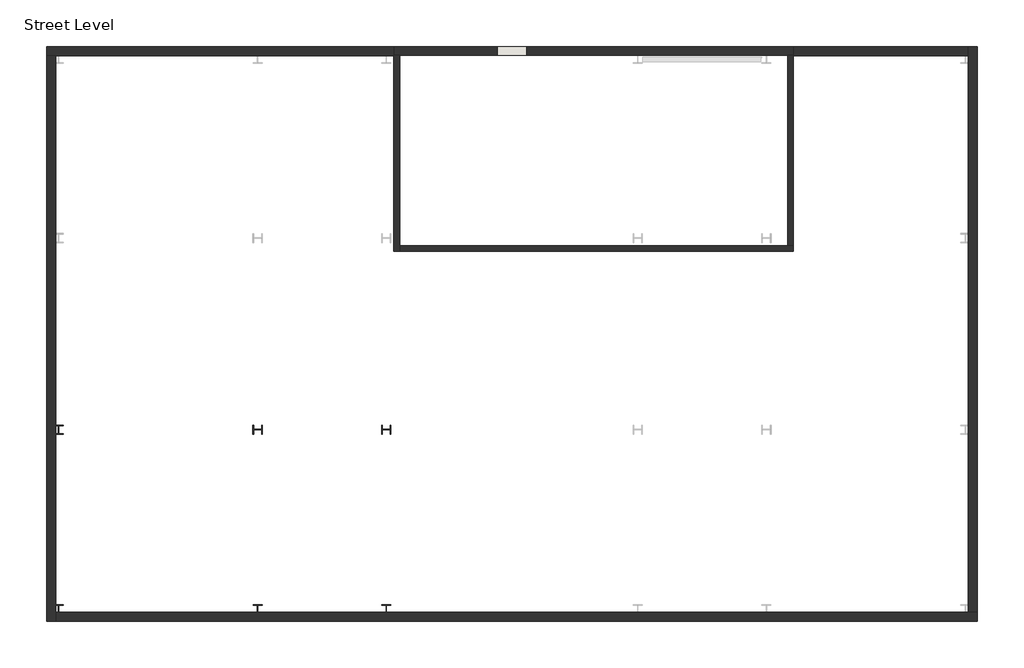
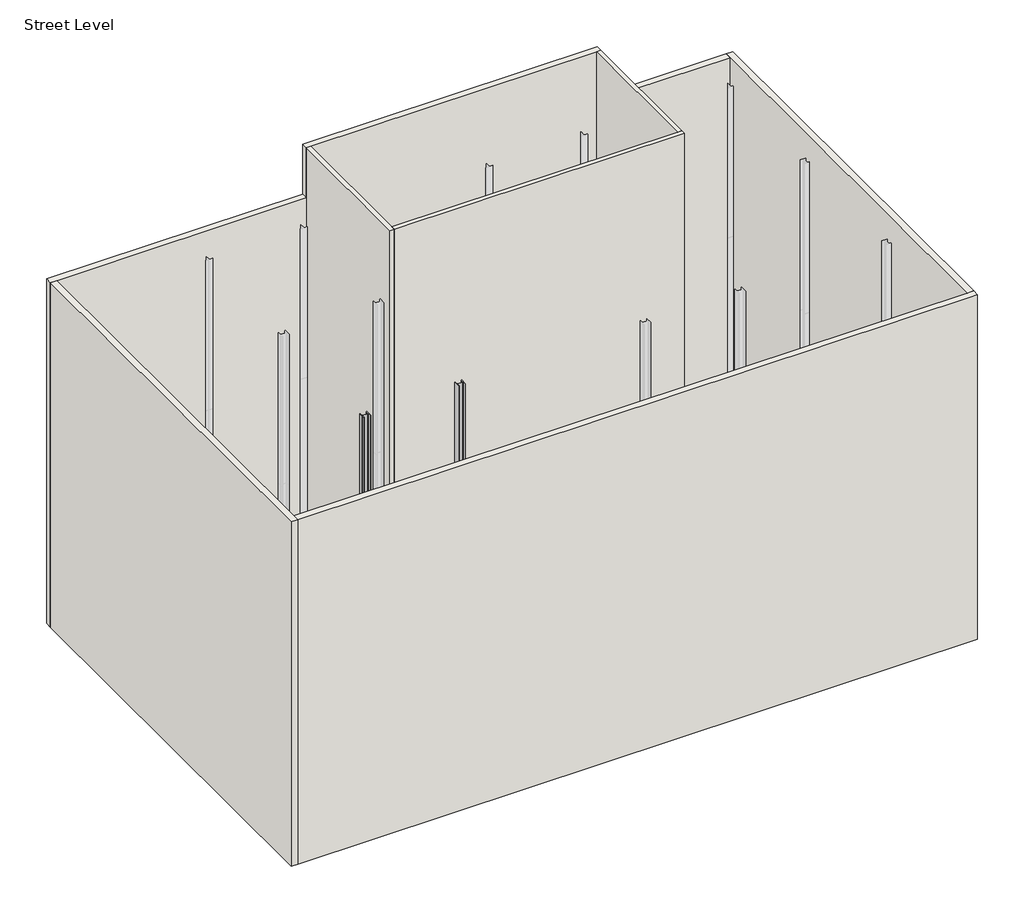
# One storey, part 1 of 3: 9 walls, 6 columns.
"""IFC4 building model written with IfcOpenShell, lengths in millimetres."""

from ifc_helpers import new_model, si_unit, point, frame, frame_2d, origin, place, context, project, spatial, polyline, circle_curve, trimmed, segment, composite_curve, outline, extrude, faceted_brep, element, save

model = new_model("IFC4")

# Units and contexts
model_context = context("Model", 3, world=origin())
ifc_project = project(units=[si_unit("LENGTHUNIT", "METRE", prefix="MILLI")], contexts=[model_context])

# Site, building, storey
site = spatial("IfcSite", under=ifc_project)
building = spatial("IfcBuilding", under=site)
storey = spatial("IfcBuildingStorey", under=building, Name="Street Level", Elevation=-914.4)

# Columns
placement = place(None, origin())
element("IfcColumn", 1, ObjectType="W-Wide Flange-Column : W12X87", at=placement, inside=storey, context=model_context, shape_type="SweptSolid", body=[
    extrude(outline(composite_curve([segment(polyline([(-9643.0622732, -3562.1684696), (-9663.6362732, -3562.1684696), (-9663.6362732, -3437.3274696)]), True, "CONTINUOUS"), segment(trimmed(circle_curve(frame_2d((-9685.9247732, -3437.3274696)), 22.2885), [point((-9663.6362732, -3437.3274696))], [point((-9685.9247732, -3415.0389696))], True, "CARTESIAN"), True, "CONTINUOUS"), segment(polyline([(-9685.9247732, -3415.0389696), (-9917.6997732, -3415.0389696)]), True, "CONTINUOUS"), segment(trimmed(circle_curve(frame_2d((-9917.6997732, -3437.3274696)), 22.2885), [point((-9917.6997732, -3415.0389696))], [point((-9939.9882732, -3437.3274696))], True, "CARTESIAN"), True, "CONTINUOUS"), segment(polyline([(-9939.9882732, -3437.3274696), (-9939.9882732, -3562.1684696), (-9960.5622732, -3562.1684696), (-9960.5622732, -3254.8284696), (-9939.9882732, -3254.8284696), (-9939.9882732, -3379.6694696)]), True, "CONTINUOUS"), segment(trimmed(circle_curve(frame_2d((-9917.6997732, -3379.6694696)), 22.2885), [point((-9939.9882732, -3379.6694696))], [point((-9917.6997732, -3401.9579696))], True, "CARTESIAN"), True, "CONTINUOUS"), segment(polyline([(-9917.6997732, -3401.9579696), (-9685.9247732, -3401.9579696)]), True, "CONTINUOUS"), segment(trimmed(circle_curve(frame_2d((-9685.9247732, -3379.6694696)), 22.2885), [point((-9685.9247732, -3401.9579696))], [point((-9663.6362732, -3379.6694696))], True, "CARTESIAN"), True, "CONTINUOUS"), segment(polyline([(-9663.6362732, -3379.6694696), (-9663.6362732, -3254.8284696), (-9643.0622732, -3254.8284696), (-9643.0622732, -3562.1684696)]), True, "CONTINUOUS")], self_intersect=False)), frame((0.0, 0.0, 7315.2), z_axis=(0.0, 0.0, 1.0), x_axis=(1.0, 0.0, 0.0)), (0.0, 0.0, 1.0), 7315.2),
    extrude(outline(composite_curve([segment(polyline([(-9643.0622732, -3562.1684696), (-9663.6362732, -3562.1684696), (-9663.6362732, -3437.3274696)]), True, "CONTINUOUS"), segment(trimmed(circle_curve(frame_2d((-9685.9247732, -3437.3274696)), 22.2885), [point((-9663.6362732, -3437.3274696))], [point((-9685.9247732, -3415.0389696))], True, "CARTESIAN"), True, "CONTINUOUS"), segment(polyline([(-9685.9247732, -3415.0389696), (-9917.6997732, -3415.0389696)]), True, "CONTINUOUS"), segment(trimmed(circle_curve(frame_2d((-9917.6997732, -3437.3274696)), 22.2885), [point((-9917.6997732, -3415.0389696))], [point((-9939.9882732, -3437.3274696))], True, "CARTESIAN"), True, "CONTINUOUS"), segment(polyline([(-9939.9882732, -3437.3274696), (-9939.9882732, -3562.1684696), (-9960.5622732, -3562.1684696), (-9960.5622732, -3254.8284696), (-9939.9882732, -3254.8284696), (-9939.9882732, -3379.6694696)]), True, "CONTINUOUS"), segment(trimmed(circle_curve(frame_2d((-9917.6997732, -3379.6694696)), 22.2885), [point((-9939.9882732, -3379.6694696))], [point((-9917.6997732, -3401.9579696))], True, "CARTESIAN"), True, "CONTINUOUS"), segment(polyline([(-9917.6997732, -3401.9579696), (-9685.9247732, -3401.9579696)]), True, "CONTINUOUS"), segment(trimmed(circle_curve(frame_2d((-9685.9247732, -3379.6694696)), 22.2885), [point((-9685.9247732, -3401.9579696))], [point((-9663.6362732, -3379.6694696))], True, "CARTESIAN"), True, "CONTINUOUS"), segment(polyline([(-9663.6362732, -3379.6694696), (-9663.6362732, -3254.8284696), (-9643.0622732, -3254.8284696), (-9643.0622732, -3562.1684696)]), True, "CONTINUOUS")], self_intersect=False)), frame((0.0, 0.0, -914.4), z_axis=(0.0, 0.0, 1.0), x_axis=(1.0, 0.0, 0.0)), (0.0, 0.0, 1.0), 8229.6),
])
element("IfcColumn", 2, ObjectType="W-Wide Flange-Column : W12X87", at=placement, inside=storey, context=model_context, shape_type="SweptSolid", body=[
    extrude(outline(composite_curve([segment(polyline([(-5274.2622732, -3562.1684696), (-5294.8362732, -3562.1684696), (-5294.8362732, -3437.3274696)]), True, "CONTINUOUS"), segment(trimmed(circle_curve(frame_2d((-5317.1247732, -3437.3274696)), 22.2885), [point((-5294.8362732, -3437.3274696))], [point((-5317.1247732, -3415.0389696))], True, "CARTESIAN"), True, "CONTINUOUS"), segment(polyline([(-5317.1247732, -3415.0389696), (-5548.8997732, -3415.0389696)]), True, "CONTINUOUS"), segment(trimmed(circle_curve(frame_2d((-5548.8997732, -3437.3274696)), 22.2885), [point((-5548.8997732, -3415.0389696))], [point((-5571.1882732, -3437.3274696))], True, "CARTESIAN"), True, "CONTINUOUS"), segment(polyline([(-5571.1882732, -3437.3274696), (-5571.1882732, -3562.1684696), (-5591.7622732, -3562.1684696), (-5591.7622732, -3254.8284696), (-5571.1882732, -3254.8284696), (-5571.1882732, -3379.6694696)]), True, "CONTINUOUS"), segment(trimmed(circle_curve(frame_2d((-5548.8997732, -3379.6694696)), 22.2885), [point((-5571.1882732, -3379.6694696))], [point((-5548.8997732, -3401.9579696))], True, "CARTESIAN"), True, "CONTINUOUS"), segment(polyline([(-5548.8997732, -3401.9579696), (-5317.1247732, -3401.9579696)]), True, "CONTINUOUS"), segment(trimmed(circle_curve(frame_2d((-5317.1247732, -3379.6694696)), 22.2885), [point((-5317.1247732, -3401.9579696))], [point((-5294.8362732, -3379.6694696))], True, "CARTESIAN"), True, "CONTINUOUS"), segment(polyline([(-5294.8362732, -3379.6694696), (-5294.8362732, -3254.8284696), (-5274.2622732, -3254.8284696), (-5274.2622732, -3562.1684696)]), True, "CONTINUOUS")], self_intersect=False)), frame((0.0, 0.0, 7315.2), z_axis=(0.0, 0.0, 1.0), x_axis=(1.0, 0.0, 0.0)), (0.0, 0.0, 1.0), 7315.2),
    extrude(outline(composite_curve([segment(polyline([(-5274.2622732, -3562.1684696), (-5294.8362732, -3562.1684696), (-5294.8362732, -3437.3274696)]), True, "CONTINUOUS"), segment(trimmed(circle_curve(frame_2d((-5317.1247732, -3437.3274696)), 22.2885), [point((-5294.8362732, -3437.3274696))], [point((-5317.1247732, -3415.0389696))], True, "CARTESIAN"), True, "CONTINUOUS"), segment(polyline([(-5317.1247732, -3415.0389696), (-5548.8997732, -3415.0389696)]), True, "CONTINUOUS"), segment(trimmed(circle_curve(frame_2d((-5548.8997732, -3437.3274696)), 22.2885), [point((-5548.8997732, -3415.0389696))], [point((-5571.1882732, -3437.3274696))], True, "CARTESIAN"), True, "CONTINUOUS"), segment(polyline([(-5571.1882732, -3437.3274696), (-5571.1882732, -3562.1684696), (-5591.7622732, -3562.1684696), (-5591.7622732, -3254.8284696), (-5571.1882732, -3254.8284696), (-5571.1882732, -3379.6694696)]), True, "CONTINUOUS"), segment(trimmed(circle_curve(frame_2d((-5548.8997732, -3379.6694696)), 22.2885), [point((-5571.1882732, -3379.6694696))], [point((-5548.8997732, -3401.9579696))], True, "CARTESIAN"), True, "CONTINUOUS"), segment(polyline([(-5548.8997732, -3401.9579696), (-5317.1247732, -3401.9579696)]), True, "CONTINUOUS"), segment(trimmed(circle_curve(frame_2d((-5317.1247732, -3379.6694696)), 22.2885), [point((-5317.1247732, -3401.9579696))], [point((-5294.8362732, -3379.6694696))], True, "CARTESIAN"), True, "CONTINUOUS"), segment(polyline([(-5294.8362732, -3379.6694696), (-5294.8362732, -3254.8284696), (-5274.2622732, -3254.8284696), (-5274.2622732, -3562.1684696)]), True, "CONTINUOUS")], self_intersect=False)), frame((0.0, 0.0, -914.4), z_axis=(0.0, 0.0, 1.0), x_axis=(1.0, 0.0, 0.0)), (0.0, 0.0, 1.0), 8229.6),
])
element("IfcColumn", 3, ObjectType="W-Wide Flange-Column : W12X87", at=placement, inside=storey, context=model_context, shape_type="SweptSolid", body=[
    extrude(outline(composite_curve([segment(polyline([(-5279.3422732, -9345.7484696), (-5279.3422732, -9366.3224696), (-5404.1832732, -9366.3224696)]), True, "CONTINUOUS"), segment(trimmed(circle_curve(frame_2d((-5404.1832732, -9388.6109696)), 22.2885), [point((-5404.1832732, -9366.3224696))], [point((-5426.4717732, -9388.6109696))], True, "CARTESIAN"), True, "CONTINUOUS"), segment(polyline([(-5426.4717732, -9388.6109696), (-5426.4717732, -9620.3859696)]), True, "CONTINUOUS"), segment(trimmed(circle_curve(frame_2d((-5404.1832732, -9620.3859696)), 22.2885), [point((-5426.4717732, -9620.3859696))], [point((-5404.1832732, -9642.6744696))], True, "CARTESIAN"), True, "CONTINUOUS"), segment(polyline([(-5404.1832732, -9642.6744696), (-5279.3422732, -9642.6744696), (-5279.3422732, -9663.2484696), (-5586.6822732, -9663.2484696), (-5586.6822732, -9642.6744696), (-5461.8412732, -9642.6744696)]), True, "CONTINUOUS"), segment(trimmed(circle_curve(frame_2d((-5461.8412732, -9620.3859696)), 22.2885), [point((-5461.8412732, -9642.6744696))], [point((-5439.5527732, -9620.3859696))], True, "CARTESIAN"), True, "CONTINUOUS"), segment(polyline([(-5439.5527732, -9620.3859696), (-5439.5527732, -9388.6109696)]), True, "CONTINUOUS"), segment(trimmed(circle_curve(frame_2d((-5461.8412732, -9388.6109696)), 22.2885), [point((-5439.5527732, -9388.6109696))], [point((-5461.8412732, -9366.3224696))], True, "CARTESIAN"), True, "CONTINUOUS"), segment(polyline([(-5461.8412732, -9366.3224696), (-5586.6822732, -9366.3224696), (-5586.6822732, -9345.7484696), (-5279.3422732, -9345.7484696)]), True, "CONTINUOUS")], self_intersect=False)), frame((0.0, 0.0, 7315.2), z_axis=(0.0, 0.0, 1.0), x_axis=(1.0, 0.0, 0.0)), (0.0, 0.0, 1.0), 7315.2),
    extrude(outline(composite_curve([segment(polyline([(-5279.3422732, -9345.7484696), (-5279.3422732, -9366.3224696), (-5404.1832732, -9366.3224696)]), True, "CONTINUOUS"), segment(trimmed(circle_curve(frame_2d((-5404.1832732, -9388.6109696)), 22.2885), [point((-5404.1832732, -9366.3224696))], [point((-5426.4717732, -9388.6109696))], True, "CARTESIAN"), True, "CONTINUOUS"), segment(polyline([(-5426.4717732, -9388.6109696), (-5426.4717732, -9620.3859696)]), True, "CONTINUOUS"), segment(trimmed(circle_curve(frame_2d((-5404.1832732, -9620.3859696)), 22.2885), [point((-5426.4717732, -9620.3859696))], [point((-5404.1832732, -9642.6744696))], True, "CARTESIAN"), True, "CONTINUOUS"), segment(polyline([(-5404.1832732, -9642.6744696), (-5279.3422732, -9642.6744696), (-5279.3422732, -9663.2484696), (-5586.6822732, -9663.2484696), (-5586.6822732, -9642.6744696), (-5461.8412732, -9642.6744696)]), True, "CONTINUOUS"), segment(trimmed(circle_curve(frame_2d((-5461.8412732, -9620.3859696)), 22.2885), [point((-5461.8412732, -9642.6744696))], [point((-5439.5527732, -9620.3859696))], True, "CARTESIAN"), True, "CONTINUOUS"), segment(polyline([(-5439.5527732, -9620.3859696), (-5439.5527732, -9388.6109696)]), True, "CONTINUOUS"), segment(trimmed(circle_curve(frame_2d((-5461.8412732, -9388.6109696)), 22.2885), [point((-5439.5527732, -9388.6109696))], [point((-5461.8412732, -9366.3224696))], True, "CARTESIAN"), True, "CONTINUOUS"), segment(polyline([(-5461.8412732, -9366.3224696), (-5586.6822732, -9366.3224696), (-5586.6822732, -9345.7484696), (-5279.3422732, -9345.7484696)]), True, "CONTINUOUS")], self_intersect=False)), frame((0.0, 0.0, -914.4), z_axis=(0.0, 0.0, 1.0), x_axis=(1.0, 0.0, 0.0)), (0.0, 0.0, 1.0), 8229.6),
])
element("IfcColumn", 4, ObjectType="W-Wide Flange-Column : W12X87", at=placement, inside=storey, context=model_context, shape_type="SweptSolid", body=[
    extrude(outline(composite_curve([segment(polyline([(-9648.1422732, -9345.7484696), (-9648.1422732, -9366.3224696), (-9772.9832732, -9366.3224696)]), True, "CONTINUOUS"), segment(trimmed(circle_curve(frame_2d((-9772.9832732, -9388.6109696)), 22.2885), [point((-9772.9832732, -9366.3224696))], [point((-9795.2717732, -9388.6109696))], True, "CARTESIAN"), True, "CONTINUOUS"), segment(polyline([(-9795.2717732, -9388.6109696), (-9795.2717732, -9620.3859696)]), True, "CONTINUOUS"), segment(trimmed(circle_curve(frame_2d((-9772.9832732, -9620.3859696)), 22.2885), [point((-9795.2717732, -9620.3859696))], [point((-9772.9832732, -9642.6744696))], True, "CARTESIAN"), True, "CONTINUOUS"), segment(polyline([(-9772.9832732, -9642.6744696), (-9648.1422732, -9642.6744696), (-9648.1422732, -9663.2484696), (-9955.4822732, -9663.2484696), (-9955.4822732, -9642.6744696), (-9830.6412732, -9642.6744696)]), True, "CONTINUOUS"), segment(trimmed(circle_curve(frame_2d((-9830.6412732, -9620.3859696)), 22.2885), [point((-9830.6412732, -9642.6744696))], [point((-9808.3527732, -9620.3859696))], True, "CARTESIAN"), True, "CONTINUOUS"), segment(polyline([(-9808.3527732, -9620.3859696), (-9808.3527732, -9388.6109696)]), True, "CONTINUOUS"), segment(trimmed(circle_curve(frame_2d((-9830.6412732, -9388.6109696)), 22.2885), [point((-9808.3527732, -9388.6109696))], [point((-9830.6412732, -9366.3224696))], True, "CARTESIAN"), True, "CONTINUOUS"), segment(polyline([(-9830.6412732, -9366.3224696), (-9955.4822732, -9366.3224696), (-9955.4822732, -9345.7484696), (-9648.1422732, -9345.7484696)]), True, "CONTINUOUS")], self_intersect=False)), frame((0.0, 0.0, 7315.2), z_axis=(0.0, 0.0, 1.0), x_axis=(1.0, 0.0, 0.0)), (0.0, 0.0, 1.0), 7315.2),
    extrude(outline(composite_curve([segment(polyline([(-9648.1422732, -9345.7484696), (-9648.1422732, -9366.3224696), (-9772.9832732, -9366.3224696)]), True, "CONTINUOUS"), segment(trimmed(circle_curve(frame_2d((-9772.9832732, -9388.6109696)), 22.2885), [point((-9772.9832732, -9366.3224696))], [point((-9795.2717732, -9388.6109696))], True, "CARTESIAN"), True, "CONTINUOUS"), segment(polyline([(-9795.2717732, -9388.6109696), (-9795.2717732, -9620.3859696)]), True, "CONTINUOUS"), segment(trimmed(circle_curve(frame_2d((-9772.9832732, -9620.3859696)), 22.2885), [point((-9795.2717732, -9620.3859696))], [point((-9772.9832732, -9642.6744696))], True, "CARTESIAN"), True, "CONTINUOUS"), segment(polyline([(-9772.9832732, -9642.6744696), (-9648.1422732, -9642.6744696), (-9648.1422732, -9663.2484696), (-9955.4822732, -9663.2484696), (-9955.4822732, -9642.6744696), (-9830.6412732, -9642.6744696)]), True, "CONTINUOUS"), segment(trimmed(circle_curve(frame_2d((-9830.6412732, -9620.3859696)), 22.2885), [point((-9830.6412732, -9642.6744696))], [point((-9808.3527732, -9620.3859696))], True, "CARTESIAN"), True, "CONTINUOUS"), segment(polyline([(-9808.3527732, -9620.3859696), (-9808.3527732, -9388.6109696)]), True, "CONTINUOUS"), segment(trimmed(circle_curve(frame_2d((-9830.6412732, -9388.6109696)), 22.2885), [point((-9808.3527732, -9388.6109696))], [point((-9830.6412732, -9366.3224696))], True, "CARTESIAN"), True, "CONTINUOUS"), segment(polyline([(-9830.6412732, -9366.3224696), (-9955.4822732, -9366.3224696), (-9955.4822732, -9345.7484696), (-9648.1422732, -9345.7484696)]), True, "CONTINUOUS")], self_intersect=False)), frame((0.0, 0.0, -914.4), z_axis=(0.0, 0.0, 1.0), x_axis=(1.0, 0.0, 0.0)), (0.0, 0.0, 1.0), 8229.6),
])
element("IfcColumn", 5, ObjectType="W-Wide Flange-Column : W12X87", at=placement, inside=storey, context=model_context, shape_type="SweptSolid", body=[
    extrude(outline(composite_curve([segment(polyline([(-16404.5422732, -9345.7484696), (-16404.5422732, -9366.3224696), (-16529.3832732, -9366.3224696)]), True, "CONTINUOUS"), segment(trimmed(circle_curve(frame_2d((-16529.3832732, -9388.6109696)), 22.2885), [point((-16529.3832732, -9366.3224696))], [point((-16551.6717732, -9388.6109696))], True, "CARTESIAN"), True, "CONTINUOUS"), segment(polyline([(-16551.6717732, -9388.6109696), (-16551.6717732, -9620.3859696)]), True, "CONTINUOUS"), segment(trimmed(circle_curve(frame_2d((-16529.3832732, -9620.3859696)), 22.2885), [point((-16551.6717732, -9620.3859696))], [point((-16529.3832732, -9642.6744696))], True, "CARTESIAN"), True, "CONTINUOUS"), segment(polyline([(-16529.3832732, -9642.6744696), (-16404.5422732, -9642.6744696), (-16404.5422732, -9663.2484696), (-16711.8822732, -9663.2484696), (-16711.8822732, -9642.6744696), (-16587.0412732, -9642.6744696)]), True, "CONTINUOUS"), segment(trimmed(circle_curve(frame_2d((-16587.0412732, -9620.3859696)), 22.2885), [point((-16587.0412732, -9642.6744696))], [point((-16564.7527732, -9620.3859696))], True, "CARTESIAN"), True, "CONTINUOUS"), segment(polyline([(-16564.7527732, -9620.3859696), (-16564.7527732, -9388.6109696)]), True, "CONTINUOUS"), segment(trimmed(circle_curve(frame_2d((-16587.0412732, -9388.6109696)), 22.2885), [point((-16564.7527732, -9388.6109696))], [point((-16587.0412732, -9366.3224696))], True, "CARTESIAN"), True, "CONTINUOUS"), segment(polyline([(-16587.0412732, -9366.3224696), (-16711.8822732, -9366.3224696), (-16711.8822732, -9345.7484696), (-16404.5422732, -9345.7484696)]), True, "CONTINUOUS")], self_intersect=False)), frame((0.0, 0.0, 7315.2), z_axis=(0.0, 0.0, 1.0), x_axis=(1.0, 0.0, 0.0)), (0.0, 0.0, 1.0), 7315.2),
    extrude(outline(composite_curve([segment(polyline([(-16404.5422732, -9345.7484696), (-16404.5422732, -9366.3224696), (-16529.3832732, -9366.3224696)]), True, "CONTINUOUS"), segment(trimmed(circle_curve(frame_2d((-16529.3832732, -9388.6109696)), 22.2885), [point((-16529.3832732, -9366.3224696))], [point((-16551.6717732, -9388.6109696))], True, "CARTESIAN"), True, "CONTINUOUS"), segment(polyline([(-16551.6717732, -9388.6109696), (-16551.6717732, -9620.3859696)]), True, "CONTINUOUS"), segment(trimmed(circle_curve(frame_2d((-16529.3832732, -9620.3859696)), 22.2885), [point((-16551.6717732, -9620.3859696))], [point((-16529.3832732, -9642.6744696))], True, "CARTESIAN"), True, "CONTINUOUS"), segment(polyline([(-16529.3832732, -9642.6744696), (-16404.5422732, -9642.6744696), (-16404.5422732, -9663.2484696), (-16711.8822732, -9663.2484696), (-16711.8822732, -9642.6744696), (-16587.0412732, -9642.6744696)]), True, "CONTINUOUS"), segment(trimmed(circle_curve(frame_2d((-16587.0412732, -9620.3859696)), 22.2885), [point((-16587.0412732, -9642.6744696))], [point((-16564.7527732, -9620.3859696))], True, "CARTESIAN"), True, "CONTINUOUS"), segment(polyline([(-16564.7527732, -9620.3859696), (-16564.7527732, -9388.6109696)]), True, "CONTINUOUS"), segment(trimmed(circle_curve(frame_2d((-16587.0412732, -9388.6109696)), 22.2885), [point((-16564.7527732, -9388.6109696))], [point((-16587.0412732, -9366.3224696))], True, "CARTESIAN"), True, "CONTINUOUS"), segment(polyline([(-16587.0412732, -9366.3224696), (-16711.8822732, -9366.3224696), (-16711.8822732, -9345.7484696), (-16404.5422732, -9345.7484696)]), True, "CONTINUOUS")], self_intersect=False)), frame((0.0, 0.0, -914.4), z_axis=(0.0, 0.0, 1.0), x_axis=(1.0, 0.0, 0.0)), (0.0, 0.0, 1.0), 8229.6),
])
element("IfcColumn", 6, ObjectType="W-Wide Flange-Column : W12X87", at=placement, inside=storey, context=model_context, shape_type="SweptSolid", body=[
    extrude(outline(composite_curve([segment(polyline([(-16404.5422732, -3249.7484696), (-16404.5422732, -3270.3224696), (-16529.3832732, -3270.3224696)]), True, "CONTINUOUS"), segment(trimmed(circle_curve(frame_2d((-16529.3832732, -3292.6109696)), 22.2885), [point((-16529.3832732, -3270.3224696))], [point((-16551.6717732, -3292.6109696))], True, "CARTESIAN"), True, "CONTINUOUS"), segment(polyline([(-16551.6717732, -3292.6109696), (-16551.6717732, -3524.3859696)]), True, "CONTINUOUS"), segment(trimmed(circle_curve(frame_2d((-16529.3832732, -3524.3859696)), 22.2885), [point((-16551.6717732, -3524.3859696))], [point((-16529.3832732, -3546.6744696))], True, "CARTESIAN"), True, "CONTINUOUS"), segment(polyline([(-16529.3832732, -3546.6744696), (-16404.5422732, -3546.6744696), (-16404.5422732, -3567.2484696), (-16711.8822732, -3567.2484696), (-16711.8822732, -3546.6744696), (-16587.0412732, -3546.6744696)]), True, "CONTINUOUS"), segment(trimmed(circle_curve(frame_2d((-16587.0412732, -3524.3859696)), 22.2885), [point((-16587.0412732, -3546.6744696))], [point((-16564.7527732, -3524.3859696))], True, "CARTESIAN"), True, "CONTINUOUS"), segment(polyline([(-16564.7527732, -3524.3859696), (-16564.7527732, -3292.6109696)]), True, "CONTINUOUS"), segment(trimmed(circle_curve(frame_2d((-16587.0412732, -3292.6109696)), 22.2885), [point((-16564.7527732, -3292.6109696))], [point((-16587.0412732, -3270.3224696))], True, "CARTESIAN"), True, "CONTINUOUS"), segment(polyline([(-16587.0412732, -3270.3224696), (-16711.8822732, -3270.3224696), (-16711.8822732, -3249.7484696), (-16404.5422732, -3249.7484696)]), True, "CONTINUOUS")], self_intersect=False)), frame((0.0, 0.0, 7315.2), z_axis=(0.0, 0.0, 1.0), x_axis=(1.0, 0.0, 0.0)), (0.0, 0.0, 1.0), 7315.2),
    extrude(outline(composite_curve([segment(polyline([(-16404.5422732, -3249.7484696), (-16404.5422732, -3270.3224696), (-16529.3832732, -3270.3224696)]), True, "CONTINUOUS"), segment(trimmed(circle_curve(frame_2d((-16529.3832732, -3292.6109696)), 22.2885), [point((-16529.3832732, -3270.3224696))], [point((-16551.6717732, -3292.6109696))], True, "CARTESIAN"), True, "CONTINUOUS"), segment(polyline([(-16551.6717732, -3292.6109696), (-16551.6717732, -3524.3859696)]), True, "CONTINUOUS"), segment(trimmed(circle_curve(frame_2d((-16529.3832732, -3524.3859696)), 22.2885), [point((-16551.6717732, -3524.3859696))], [point((-16529.3832732, -3546.6744696))], True, "CARTESIAN"), True, "CONTINUOUS"), segment(polyline([(-16529.3832732, -3546.6744696), (-16404.5422732, -3546.6744696), (-16404.5422732, -3567.2484696), (-16711.8822732, -3567.2484696), (-16711.8822732, -3546.6744696), (-16587.0412732, -3546.6744696)]), True, "CONTINUOUS"), segment(trimmed(circle_curve(frame_2d((-16587.0412732, -3524.3859696)), 22.2885), [point((-16587.0412732, -3546.6744696))], [point((-16564.7527732, -3524.3859696))], True, "CARTESIAN"), True, "CONTINUOUS"), segment(polyline([(-16564.7527732, -3524.3859696), (-16564.7527732, -3292.6109696)]), True, "CONTINUOUS"), segment(trimmed(circle_curve(frame_2d((-16587.0412732, -3292.6109696)), 22.2885), [point((-16564.7527732, -3292.6109696))], [point((-16587.0412732, -3270.3224696))], True, "CARTESIAN"), True, "CONTINUOUS"), segment(polyline([(-16587.0412732, -3270.3224696), (-16711.8822732, -3270.3224696), (-16711.8822732, -3249.7484696), (-16404.5422732, -3249.7484696)]), True, "CONTINUOUS")], self_intersect=False)), frame((0.0, 0.0, -914.4), z_axis=(0.0, 0.0, 1.0), x_axis=(1.0, 0.0, 0.0)), (0.0, 0.0, 1.0), 8229.6),
])

# Walls
element("IfcWall", 7, ObjectType="Generic - 12\"", at=placement, inside=storey, context=model_context, shape_type="Brep", body=[
    faceted_brep([(-16964.6122732, 9291.5015304, -914.4), (-16659.8122732, 9291.5015304, -914.4), (-5174.2497732, 9291.5015304, -914.4), (-5174.2497732, 9291.5015304, 0.0), (-5174.2497732, 9291.5015304, 3657.6), (-5174.2497732, 9291.5015304, 7315.2), (-5174.2497732, 9291.5015304, 10972.8), (-5174.2497732, 9291.5015304, 14630.4), (-5174.2497732, 9291.5015304, 15849.6), (-16659.8122732, 9291.5015304, 15849.6), (-16964.6122732, 9291.5015304, 15849.6), (-16964.6122732, 9596.3015304, -914.4), (-16964.6122732, 9596.3015304, 15849.6), (-5174.2497732, 9596.3015304, 15849.6), (-5174.2497732, 9596.3015304, -914.4)], [[[0, 1, 2, 3, 4, 5, 6, 7, 8, 9, 10]], [[11, 12, 13, 14]], [[2, 1, 0, 11, 14]], [[10, 9, 8, 13, 12]], [[0, 10, 12, 11]], [[8, 7, 6, 5, 4, 3, 2, 14, 13]]]),
])
element("IfcWall", 8, ObjectType="Generic - 12\"", at=placement, inside=storey, context=model_context, shape_type="Brep", body=[
    faceted_brep([(-16659.8122732, -9910.8984696, -914.4), (-16659.8122732, -9606.0984696, -914.4), (-16659.8122732, 9291.5015304, -914.4), (-16659.8122732, 9291.5015304, 0.0), (-16659.8122732, 9291.5015304, 3657.6), (-16659.8122732, 9291.5015304, 7010.4), (-16659.8122732, 9291.5015304, 7315.2), (-16659.8122732, 9291.5015304, 10972.8), (-16659.8122732, 9291.5015304, 14630.4), (-16659.8122732, 9291.5015304, 15849.6), (-16659.8122732, -9606.0984696, 15849.6), (-16659.8122732, -9910.8984696, 15849.6), (-16964.6122732, -9910.8984696, -914.4), (-16964.6122732, -9910.8984696, 15849.6), (-16964.6122732, 9291.5015304, 15849.6), (-16964.6122732, 9291.5015304, -914.4)], [[[0, 1, 2, 3, 4, 5, 6, 7, 8, 9, 10, 11]], [[12, 13, 14, 15]], [[2, 1, 0, 12, 15]], [[11, 10, 9, 14, 13]], [[0, 11, 13, 12]], [[9, 8, 7, 6, 5, 4, 3, 2, 15, 14]]]),
])
element("IfcWall", 9, ObjectType="Generic - 12\"", at=placement, inside=storey, context=model_context, shape_type="Brep", body=[
    faceted_brep([(14632.9877268, -9606.0984696, -914.4), (14328.1877268, -9606.0984696, -914.4), (-16659.8122732, -9606.0984696, -914.4), (-16659.8122732, -9606.0984696, 0.0), (-16659.8122732, -9606.0984696, 3657.6), (-16659.8122732, -9606.0984696, 7010.4), (-16659.8122732, -9606.0984696, 7315.2), (-16659.8122732, -9606.0984696, 10972.8), (-16659.8122732, -9606.0984696, 14630.4), (-16659.8122732, -9606.0984696, 15849.6), (14328.1877268, -9606.0984696, 15849.6), (14632.9877268, -9606.0984696, 15849.6), (14632.9877268, -9910.8984696, -914.4), (14632.9877268, -9910.8984696, 15849.6), (-16659.8122732, -9910.8984696, 15849.6), (-16659.8122732, -9910.8984696, -914.4)], [[[0, 1, 2, 3, 4, 5, 6, 7, 8, 9, 10, 11]], [[12, 13, 14, 15]], [[2, 1, 0, 12, 15]], [[11, 10, 9, 14, 13]], [[0, 11, 13, 12]], [[9, 8, 7, 6, 5, 4, 3, 2, 15, 14]]]),
])
element("IfcWall", 10, ObjectType="Generic - 12\"", at=placement, inside=storey, context=model_context, shape_type="Brep", body=[
    faceted_brep([(14328.1877268, 9596.3015304, -914.4), (14328.1877268, 9291.5015304, -914.4), (14328.1877268, -9606.0984696, -914.4), (14328.1877268, -9606.0984696, 0.0), (14328.1877268, -9606.0984696, 3657.6), (14328.1877268, -9606.0984696, 7010.4), (14328.1877268, -9606.0984696, 7315.2), (14328.1877268, -9606.0984696, 10972.8), (14328.1877268, -9606.0984696, 14630.4), (14328.1877268, -9606.0984696, 15849.6), (14328.1877268, 9291.5015304, 15849.6), (14328.1877268, 9596.3015304, 15849.6), (14632.9877268, 9596.3015304, -914.4), (14632.9877268, 9596.3015304, 15849.6), (14632.9877268, -9606.0984696, 15849.6), (14632.9877268, -9606.0984696, -914.4)], [[[0, 1, 2, 3, 4, 5, 6, 7, 8, 9, 10, 11]], [[12, 13, 14, 15]], [[2, 1, 0, 12, 15]], [[11, 10, 9, 14, 13]], [[0, 11, 13, 12]], [[9, 8, 7, 6, 5, 4, 3, 2, 15, 14]]]),
])
element("IfcWall", 11, ObjectType="Generic - 12\"", at=placement, inside=storey, context=model_context, shape_type="SweptSolid", body=[
    extrude(outline(polyline([(14328.1877268, 9291.5015304), (8379.8252268, 9291.5015304), (8379.8252268, 9596.3015304), (14328.1877268, 9596.3015304), (14328.1877268, 9291.5015304)])), frame((0.0, 0.0, -914.4), z_axis=(0.0, 0.0, 1.0), x_axis=(1.0, 0.0, 0.0)), (0.0, 0.0, 1.0), 16764.0),
])
element("IfcWall", 12, ObjectType="Generic - 12\" Masonry", at=placement, inside=storey, context=model_context, shape_type="Brep", body=[
    faceted_brep([(-5174.2497732, 9301.0265304, 18288.0), (-5174.2497732, 9301.0265304, -914.4), (-4980.5747732, 9301.0265304, -914.4), (8186.1502268, 9301.0265304, -914.4), (8379.8252268, 9301.0265304, -914.4), (8379.8252268, 9301.0265304, 18288.0), (8186.1502268, 9301.0265304, 18288.0), (-4980.5747732, 9301.0265304, 18288.0), (-1673.8122732, 9301.0265304, 0.0), (-1673.8122732, 9301.0265304, 2235.2), (-657.8122732, 9301.0265304, 2235.2), (-657.8122732, 9301.0265304, 0.0), (-5174.2497732, 9596.3015304, -914.4), (-5174.2497732, 9596.3015304, 18288.0), (8379.8252268, 9596.3015304, 18288.0), (8379.8252268, 9596.3015304, -914.4), (-1673.8122732, 9596.3015304, 0.0), (-657.8122732, 9596.3015304, 0.0), (-657.8122732, 9596.3015304, 2235.2), (-1673.8122732, 9596.3015304, 2235.2)], [[[0, 1, 2, 3, 4, 5, 6, 7], [8, 9, 10, 11]], [[12, 13, 14, 15], [16, 17, 18, 19]], [[4, 3, 2, 1, 12, 15]], [[0, 7, 6, 5, 14, 13]], [[8, 11, 17, 16]], [[11, 10, 18, 17]], [[10, 9, 19, 18]], [[9, 8, 16, 19]], [[0, 13, 12, 1]], [[4, 15, 14, 5]]]),
])
element("IfcWall", 13, ObjectType="Generic - 8\" Masonry", at=placement, inside=storey, context=model_context, shape_type="Brep", body=[
    faceted_brep([(-5174.2497732, 9301.0265304, 18288.0), (-5174.2497732, 9301.0265304, 14630.4), (-5174.2497732, 9301.0265304, 10972.8), (-5174.2497732, 9301.0265304, 7315.2), (-5174.2497732, 9301.0265304, 3657.6), (-5174.2497732, 9301.0265304, 0.0), (-5174.2497732, 9301.0265304, -914.4), (-5174.2497732, 2641.4640304, -914.4), (-5174.2497732, 2641.4640304, 18288.0), (-4980.5747732, 9301.0265304, -914.4), (-4980.5747732, 9301.0265304, 18288.0), (-4980.5747732, 2835.1390304, 18288.0), (-4980.5747732, 2641.4640304, 18288.0), (-4980.5747732, 2641.4640304, -914.4), (-4980.5747732, 2835.1390304, -914.4)], [[[0, 1, 2, 3, 4, 5, 6, 7, 8]], [[9, 10, 11, 12, 13, 14]], [[7, 6, 9, 14, 13]], [[0, 8, 12, 11, 10]], [[8, 7, 13, 12]], [[0, 10, 9, 6, 5, 4, 3, 2, 1]]]),
])
element("IfcWall", 14, ObjectType="Generic - 8\" Masonry", at=placement, inside=storey, context=model_context, shape_type="Brep", body=[
    faceted_brep([(8379.8252268, 2835.1390304, -914.4), (8186.1502268, 2835.1390304, -914.4), (-4980.5747732, 2835.1390304, -914.4), (-4980.5747732, 2835.1390304, 18288.0), (8186.1502268, 2835.1390304, 18288.0), (8379.8252268, 2835.1390304, 18288.0), (8379.8252268, 2641.4640304, -914.4), (8379.8252268, 2641.4640304, 18288.0), (-4980.5747732, 2641.4640304, 18288.0), (-4980.5747732, 2641.4640304, -914.4)], [[[0, 1, 2, 3, 4, 5]], [[6, 7, 8, 9]], [[2, 1, 0, 6, 9]], [[5, 4, 3, 8, 7]], [[3, 2, 9, 8]], [[0, 5, 7, 6]]]),
])
element("IfcWall", 15, ObjectType="Generic - 8\" Masonry", at=placement, inside=storey, context=model_context, shape_type="SweptSolid", body=[
    extrude(outline(polyline([(8186.1502268, 2835.1390304), (8186.1502268, 9301.0265304), (8379.8252268, 9301.0265304), (8379.8252268, 2835.1390304), (8186.1502268, 2835.1390304)])), frame((0.0, 0.0, -914.4), z_axis=(0.0, 0.0, 1.0), x_axis=(1.0, 0.0, 0.0)), (0.0, 0.0, 1.0), 19202.4),
])

save(model, "model.ifc")

# Revit data of these elements
# Project information
#   Organization Name = "G3B Press"
#   Organization Description = "Paul F. Aubin Cosulting Services, Inc."
#   Building Name = "Revit Essentials for Architecture"
#   Author = "Paul F. Aubin"
#   Author Website = "https://www.paulaubin.com"
#   Copyright = "Copyright © 2020 Paul F Aubin, all rights reserved"
#   Project Issue Date = "8/1/2020"
#   Project Status = "Design Development"
#   Client Name = "Groups and Links"
#   Project Address = "123 State ST\nSuite 301\nChicago, IL 60606"
#   Project Name = "07 Commercial"
#   Project Number = "2020.04A"
# Grids (mm)
#   "1": line (-22547.601, -9504.498) -> (19277.595, -9504.498)
#   "2": line (-22547.601, -3408.498) -> (19277.595, -3408.498)
#   "3": line (-22547.601, 3093.902) -> (19277.595, 3093.902)
#   "4": line (-22547.601, 9189.902) -> (19277.595, 9189.902)
#   "A": line (-16558.212, 12259.726) -> (-16558.212, -14197.104)
#   "B": line (-9801.812, 12259.726) -> (-9801.812, -14197.104)
#   "C": line (-5433.012, 12259.726) -> (-5433.012, -14197.104)
#   "D": line (3101.388, 12259.726) -> (3101.388, -14197.104)
#   "E": line (7470.188, 12259.726) -> (7470.188, -14197.104)
#   "F": line (14226.588, 12259.726) -> (14226.588, -14197.104)
#   "C.3": line (-2689.812, -15151.11) -> (-2689.812, -5965.346)
#   "C.7": line (358.188, -15151.11) -> (358.188, -5965.346)
# Type "W-Wide Flange-Column : W12X87"
#   Assembly Code = "B10"
#   W = 87
#   bf = 1' - 0.1"
#   d = 1' - 0 1/2"
#   k = 0' - 1 11/16"
#   kr = 0' - 0.8775"
#   tf = 0' - 0.81"
#   tw = 0' - 0.515"
#   A = 0.177778 SF
#   Structural Material [instance default] = Steel ASTM A992
# Type "Generic - 12\""
#   Assembly Code = "B2010"
#   Layers, outside or top first: 1' - 0" no material (function 1)
# Type "Generic - 12\" Masonry"
#   Assembly Code = "B2010"
#   Layers, outside or top first: 0' - 11 5/8" "Concrete Masonry Units" (function 1)
# Type "Generic - 8\" Masonry"
#   Assembly Code = "B2010"
#   Layers, outside or top first: 0' - 7 5/8" "Concrete Masonry Units" (function 1)
# Elements 1, 2, 3, 4, 5, 6 (IfcColumn, "W-Wide Flange-Column : W12X87")
#   Structural Material = Steel ASTM A992
#   Phase Created = New Construction
#   Materials on its faces: "Steel ASTM A992"
# Elements 7, 8, 9, 10, 11 (IfcWall, "Generic - 12\"")
#   Top Offset = 4' - 0"
#   Base Offset = 0' - 0"
#   wall height = 55' - 0"
#   Phase Created = New Construction
#   Base Constraint = Street Level
#   Top Constraint = Roof
#   Materials on its faces: "Default Wall"
# Element 12 (IfcWall, "Generic - 12\" Masonry")
#   Top Offset = 12' - 0"
#   Base Offset = 0' - 0"
#   wall height = 63' - 0"
#   Phase Created = New Construction
#   Base Constraint = Street Level
#   Top Constraint = Roof
#   Materials on its faces: "Concrete Masonry Units"
# Elements 13, 14, 15 (IfcWall, "Generic - 8\" Masonry")
#   Comments = ""
#   Top Offset = 12' - 0"
#   Base Offset = 0' - 0"
#   wall height = 63' - 0"
#   Phase Created = New Construction
#   Base Constraint = Street Level
#   Top Constraint = Roof
#   Materials on its faces: "Concrete Masonry Units"
# Materials
#   "Steel ASTM A992": class "Metal", colour RGB 199 199 199, transparency 0, Description = "Structural steel 50ksi", Cost = 0
#   "Concrete Masonry Units": class "Masonry", colour RGB 227 227 227, transparency 0, Description = "Concrete masonry units", Cost = 0
#   "Default Wall": class "Miscellaneous", colour RGB 128 128 128, transparency 0, Cost = 0
